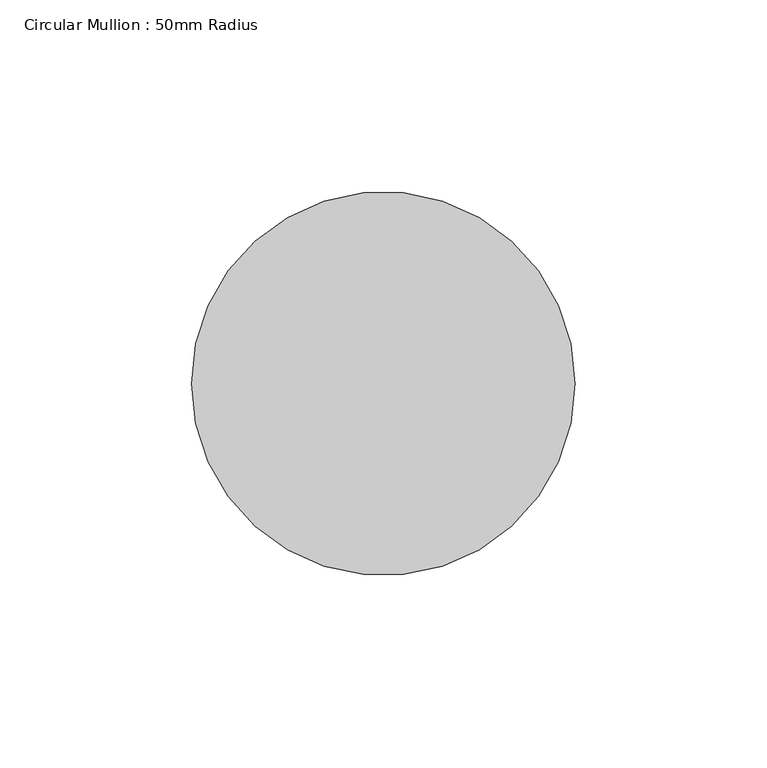
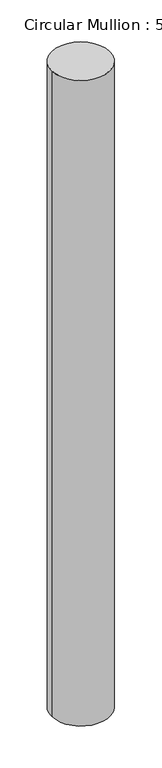
"""IFC4 building model written with IfcOpenShell, lengths in millimetres: member geometry, Circular Mullion : 50mm Radius."""

from ifc_helpers import new_model, si_unit, point, frame, origin, origin_2d, place, context, project, spatial, circle_curve, trimmed, segment, composite_curve, outline, extrude, source, transform, mapped, element, save


def circular_mullion_50mm_radius_cfc24594(model_context):
    return source(origin(), model_context, "Body", "SweptSolid", [
        extrude(outline(composite_curve([segment(trimmed(circle_curve(origin_2d(), 50.0), [point((50.0, 0.0))], [point((-50.0, 0.0))], False, "CARTESIAN"), True, "CONTINUOUS"), segment(trimmed(circle_curve(origin_2d(), 50.0), [point((-50.0, 0.0))], [point((50.0, 0.0))], False, "CARTESIAN"), True, "CONTINUOUS")], self_intersect=False)), frame((0.0, 0.0, -1174.2324107), z_axis=(0.0, 0.0, 1.0), x_axis=(1.0, 0.0, 0.0)), (0.0, 0.0, 1.0), 1174.2324107),
    ])


if __name__ == "__main__":
    model = new_model("IFC4")
    model_context = context("Model", 3, world=origin())
    ifc_project = project(units=[si_unit("LENGTHUNIT", "METRE", prefix="MILLI")], contexts=[model_context])
    site = spatial("IfcSite", under=ifc_project)
    building = spatial("IfcBuilding", under=site)
    placement = place(None, origin())
    circular_mullion_50mm_radius_shape = circular_mullion_50mm_radius_cfc24594(model_context)
    element("IfcMember", 1, ObjectType="Circular Mullion : 50mm Radius", at=placement, inside=building, context=model_context, shape_type="MappedRepresentation", body=[
        mapped(circular_mullion_50mm_radius_shape, transform((0.0, 0.0, 0.0), x_axis=(1.0, 0.0, 0.0), y_axis=(0.0, 1.0, 0.0), z_axis=(0.0, 0.0, 1.0))),
    ])
    save(model, "model.ifc")

# Revit data of these elements
# Type "Circular Mullion : 50mm Radius"
#   built-in parameter 1007350 = 0.164042 (stored number, unit not read)
# Element 1 (IfcMember, "Circular Mullion : 50mm Radius")
#   Materials on its faces: "Aluminium"
# Materials
#   "Aluminium": class "Metal", colour RGB 247 247 247, transparency 0, Description = "Aluminium 6061", Cost = 0
